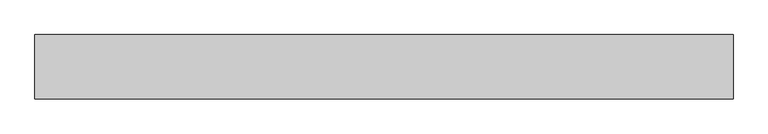
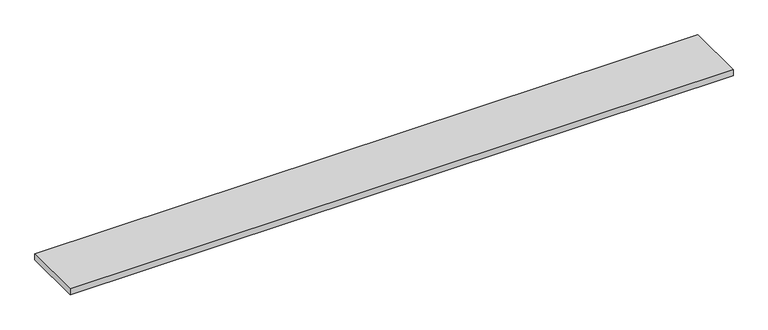
"""IFC4 building model written with IfcOpenShell, lengths in millimetres: proxy geometry, Plywood panel002 3396 : Plywood panel002 3396."""

import ifcopenshell
import ifcopenshell.guid

model = None  # the IFC model being written
_history = None  # IfcOwnerHistory: only IFC2X3 demands one
_inside = {}  # id of a spatial element -> (the spatial element, [elements in it])
_under = {}  # id of a project, library or spatial element -> (it, [spatial elements below it])
_declared = {}  # id of a project -> (the project, [libraries it declares])
_typed = {}  # id of a type object -> (the type object, [elements of that type])
_made_of = {}  # id of a material, layer set ... -> (it, [elements and type objects made of it])


def new_model(schema):
    """Start an empty IFC model of exactly this schema.

    Asked for "IFC4X3", IfcOpenShell would pick the latest addendum, in which some entities
    have other attributes; the version numbers below select the first issue.
    IFC2X3 requires an IfcOwnerHistory on every rooted entity: one is made here for all.
    """
    global model, _history
    if schema == "IFC4X3":
        model = ifcopenshell.file(schema_version=(4, 3, 0, 0))
    else:
        model = ifcopenshell.file(schema=schema)
    _inside.clear()
    _under.clear()
    _declared.clear()
    _typed.clear()
    _made_of.clear()
    _history = None
    if model.schema == "IFC2X3":
        org = make("IfcOrganization", Name="unknown")
        user = make(
            "IfcPersonAndOrganization",
            ThePerson=make("IfcPerson", FamilyName="unknown"),
            TheOrganization=org,
        )
        app = make(
            "IfcApplication",
            ApplicationDeveloper=org,
            Version="unknown",
            ApplicationFullName="unknown",
            ApplicationIdentifier="unknown",
        )
        _history = make(
            "IfcOwnerHistory",
            OwningUser=user,
            OwningApplication=app,
            ChangeAction="ADDED",
            CreationDate=0,
        )
    return model


def make(cls, **values):
    """One entity of the class cls with the attributes given. An attribute that is None is left unset."""
    return model.create_entity(
        cls, **{name: value for name, value in values.items() if value is not None}
    )


def rooted(cls, **values):
    """An entity with a GlobalId (a new one), such as an element, a storey or a relation."""
    return make(cls, GlobalId=ifcopenshell.guid.new(), OwnerHistory=_history, **values)


def si_unit(unit_type, name, prefix=None):
    """IfcSIUnit, for example si_unit("LENGTHUNIT", "METRE", prefix="MILLI")."""
    return make("IfcSIUnit", UnitType=unit_type, Prefix=prefix, Name=name)


def assignment(units):
    """IfcUnitAssignment: the units of a project."""
    return None if units is None else make("IfcUnitAssignment", Units=units)


def point(xyz):
    """IfcCartesianPoint."""
    return None if xyz is None else make("IfcCartesianPoint", Coordinates=xyz)


def direction(xyz):
    """IfcDirection."""
    return None if xyz is None else make("IfcDirection", DirectionRatios=xyz)


def frame(location, z_axis=None, x_axis=None):
    """IfcAxis2Placement3D, a coordinate frame: its origin and axes. An axis left out is left unset."""
    return make(
        "IfcAxis2Placement3D",
        Location=point(location),
        Axis=direction(z_axis),
        RefDirection=direction(x_axis),
    )


def origin():
    """The frame at (0, 0, 0) with its axes left unset."""
    return frame((0.0, 0.0, 0.0))


def place(relative_to, where):
    """IfcLocalPlacement: puts the frame where relative to a parent placement (None: the world)."""
    return make(
        "IfcLocalPlacement", PlacementRelTo=relative_to, RelativePlacement=where
    )


def context(
    kind, dimensions, precision=None, world=None, true_north=None, identifier=None
):
    """IfcGeometricRepresentationContext, for example the 3D "Model" context."""
    return make(
        "IfcGeometricRepresentationContext",
        ContextIdentifier=identifier,
        ContextType=kind,
        CoordinateSpaceDimension=dimensions,
        Precision=precision,
        WorldCoordinateSystem=world,
        TrueNorth=true_north,
    )


def project(units=None, contexts=None):
    """IfcProject with its units and contexts."""
    return rooted(
        "IfcProject",
        Name="project",
        RepresentationContexts=contexts,
        UnitsInContext=assignment(units),
    )


def spatial(cls, under=None, at=None, **own):
    """A site, building, storey or space (cls), placed at a placement, below another one or the project."""
    s = rooted(cls, ObjectPlacement=at, **own)
    if under is not None:
        _under.setdefault(under.id(), (under, []))[1].append(s)
    return s


def polyline(points):
    """IfcPolyline through the points."""
    return make("IfcPolyline", Points=[point(p) for p in points])


def outline(outer, holes=None, kind="AREA"):
    """IfcArbitraryClosedProfileDef: a profile drawn as a closed curve; with holes, ...WithVoids."""
    if holes is None:
        return make("IfcArbitraryClosedProfileDef", ProfileType=kind, OuterCurve=outer)
    return make(
        "IfcArbitraryProfileDefWithVoids",
        ProfileType=kind,
        OuterCurve=outer,
        InnerCurves=holes,
    )


def extrude(swept, where, along, depth):
    """IfcExtrudedAreaSolid: the profile swept, set in the frame where, extruded along a direction by depth."""
    return make(
        "IfcExtrudedAreaSolid",
        SweptArea=swept,
        Position=where,
        ExtrudedDirection=direction(along),
        Depth=depth,
    )


def shape(context_of_items, identifier, shape_type, items):
    """IfcShapeRepresentation: the items that make up one representation, for example the "Body"."""
    return make(
        "IfcShapeRepresentation",
        ContextOfItems=context_of_items,
        RepresentationIdentifier=identifier,
        RepresentationType=shape_type,
        Items=items,
    )


def source(mapping_origin, context_of_items, identifier, shape_type, items):
    """IfcRepresentationMap: a shape defined once, which mapped items show again and again."""
    return make(
        "IfcRepresentationMap",
        MappingOrigin=mapping_origin,
        MappedRepresentation=shape(context_of_items, identifier, shape_type, items),
    )


def transform(
    local_origin,
    x_axis=None,
    y_axis=None,
    z_axis=None,
    scale=None,
    scale2=None,
    scale3=None,
    uniform=True,
):
    """IfcCartesianTransformationOperator3D, or its non-uniform kind. x_axis, y_axis, z_axis: its Axis1, 2, 3."""
    if uniform:
        return make(
            "IfcCartesianTransformationOperator3D",
            Axis1=direction(x_axis),
            Axis2=direction(y_axis),
            LocalOrigin=point(local_origin),
            Scale=scale,
            Axis3=direction(z_axis),
        )
    return make(
        "IfcCartesianTransformationOperator3DnonUniform",
        Axis1=direction(x_axis),
        Axis2=direction(y_axis),
        LocalOrigin=point(local_origin),
        Scale=scale,
        Axis3=direction(z_axis),
        Scale2=scale2,
        Scale3=scale3,
    )


def mapped(mapping_source, mapping_target):
    """IfcMappedItem: shows the shape of a source again, moved by a transform."""
    return make(
        "IfcMappedItem", MappingSource=mapping_source, MappingTarget=mapping_target
    )


def made_of(thing, what):
    """Note that an element or type object is made of a material, layer set ...; save() writes the relation."""
    if what is not None:
        _made_of.setdefault(what.id(), (what, []))[1].append(thing)
    return thing


def element(
    cls,
    number,
    at=None,
    inside=None,
    cuts=None,
    type_object=None,
    material=None,
    context=None,
    identifier="Body",
    shape_type=None,
    held_by="IfcProductDefinitionShape",
    body=None,
    shapes=None,
    **own,
):
    """One element of the class cls, such as IfcWall. Its Tag is "e" and its number.

    at: its placement. inside: the storey or other place that contains it. cuts: it is an
    opening in that element (IfcRelVoidsElement). A single representation is given by context,
    identifier, shape_type and body (its items); several are given by shapes. held_by: the class
    of the entity that holds the representations. save() writes the other relations.
    """
    e = rooted(cls, Tag="e%d" % number, ObjectPlacement=at, **own)
    if body is not None:
        shapes = [shape(context, identifier, shape_type, body)]
    if shapes is not None:
        e.Representation = make(held_by, Representations=shapes)
    if inside is not None:
        _inside.setdefault(inside.id(), (inside, []))[1].append(e)
    if cuts is not None:
        rooted(
            "IfcRelVoidsElement", RelatingBuildingElement=cuts, RelatedOpeningElement=e
        )
    if type_object is not None:
        _typed.setdefault(type_object.id(), (type_object, []))[1].append(e)
    return made_of(e, material)


def aggregate(whole, parts):
    """IfcRelAggregates: a whole, such as a stair, and the parts it consists of."""
    return rooted("IfcRelAggregates", RelatingObject=whole, RelatedObjects=parts)


def save(model, path):
    """Write the relations noted so far, then the file.

    IfcRelAggregates (storeys below a building ...), IfcRelContainedInSpatialStructure (elements
    in a storey), IfcRelDefinesByType, IfcRelAssociatesMaterial and IfcRelDeclares: one each for
    every whole, place, type object, material and project.
    """
    for whole, parts in _under.values():
        aggregate(whole, parts)
    for where, things in _inside.values():
        rooted(
            "IfcRelContainedInSpatialStructure",
            RelatedElements=things,
            RelatingStructure=where,
        )
    for kind, things in _typed.values():
        rooted("IfcRelDefinesByType", RelatedObjects=things, RelatingType=kind)
    for what, things in _made_of.values():
        rooted("IfcRelAssociatesMaterial", RelatedObjects=things, RelatingMaterial=what)
    for by, libraries in _declared.values():
        rooted("IfcRelDeclares", RelatingContext=by, RelatedDefinitions=libraries)
    model.write(path)


def generic_models_265cc60e(model_context):
    return source(origin(), model_context, "Body", "SweptSolid", [
        extrude(outline(polyline([(3694.2883192, 10233.5750834), (3694.2883192, 10417.7250834), (5694.2883192, 10417.7250834), (5694.2883192, 10233.5750834), (3694.2883192, 10233.5750834)])), frame((0.0, 0.0, 39420.546), z_axis=(0.0, 0.0, 1.0), x_axis=(1.0, 0.0, 0.0)), (0.0, 0.0, 1.0), 19.05),
    ])


if __name__ == "__main__":
    model = new_model("IFC4")
    model_context = context("Model", 3, world=origin())
    ifc_project = project(units=[si_unit("LENGTHUNIT", "METRE", prefix="MILLI")], contexts=[model_context])
    site = spatial("IfcSite", under=ifc_project)
    building = spatial("IfcBuilding", under=site)
    placement = place(None, origin())
    generic_models_shape = generic_models_265cc60e(model_context)
    element("IfcBuildingElementProxy", 1, Name="Plywood panel002 3396 : Plywood panel002 3396", ObjectType="Plywood panel002 3396 : Plywood panel002 3396", at=placement, inside=building, context=model_context, shape_type="MappedRepresentation", body=[
        mapped(generic_models_shape, transform((0.0, 0.0, 0.0), x_axis=(1.0, 0.0, 0.0), y_axis=(0.0, 1.0, 0.0), z_axis=(0.0, 0.0, 1.0))),
    ])
    save(model, "model.ifc")

# Revit data of these elements
# Type "Plywood panel002 3396 : Plywood panel002 3396"
#   NameOverride = "Plywood panel002"
# Element 1 (IfcBuildingElementProxy, "Plywood panel002 3396 : Plywood panel002 3396")
#   Materials on its faces: "CDX PLYWOOD -  SEE STRUCTURAL DWGS"
# Materials
#   "CDX PLYWOOD -  SEE STRUCTURAL DWGS": class "Unassigned", colour RGB 177 130 114, transparency 0, Cost = 0
